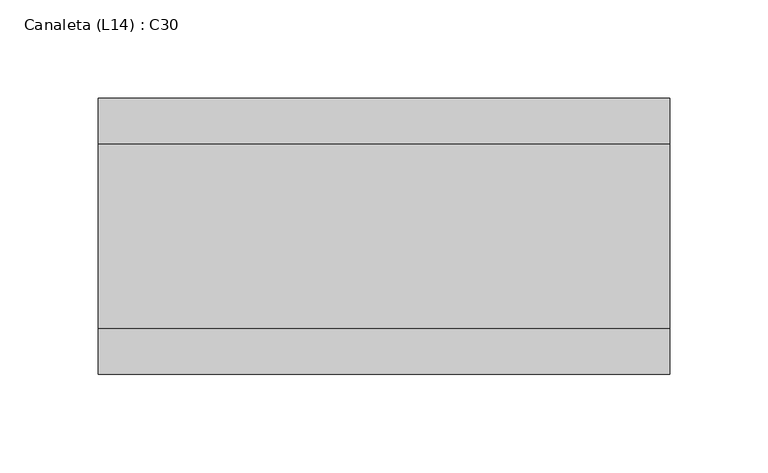
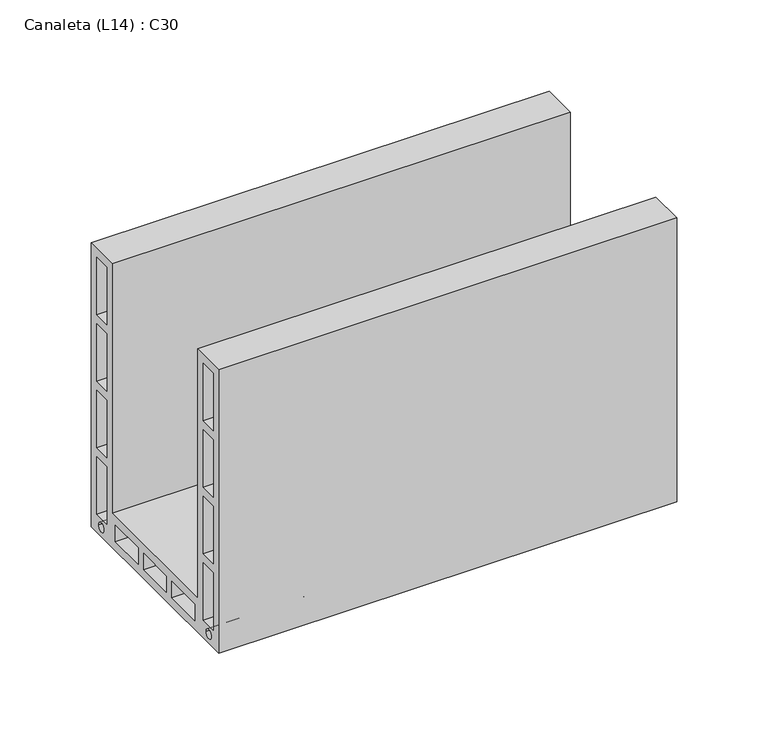
"""IFC4 building model written with IfcOpenShell, lengths in millimetres: proxy geometry, Canaleta (L14) : C30."""

from ifc_helpers import new_model, si_unit, point, frame, frame_2d, origin, place, context, project, spatial, polyline, circle_curve, trimmed, segment, composite_curve, outline, extrude, source, transform, mapped, element, save


def canaleta_l14_c30_f4fa639d(model_context):
    return source(origin(), model_context, "Body", "SweptSolid", [
        extrude(outline(polyline([(-140.0, 0.0), (-140.0, 190.0), (-117.0, 190.0), (-117.0, 23.0), (-23.0, 23.0), (-23.0, 190.0), (0.0, 190.0), (0.0, 0.0), (-140.0, 0.0)]), holes=[polyline([(-123.0, 184.0), (-134.0, 184.0), (-134.0, 145.5), (-123.0, 145.5), (-123.0, 184.0)]), polyline([(-123.0, 139.5), (-134.0, 139.5), (-134.0, 101.0), (-123.0, 101.0), (-123.0, 139.5)]), polyline([(-123.0, 95.0), (-134.0, 95.0), (-134.0, 56.5), (-123.0, 56.5), (-123.0, 95.0)]), polyline([(-123.0, 50.5), (-134.0, 50.5), (-134.0, 12.0), (-123.0, 12.0), (-123.0, 50.5)]), composite_curve([segment(trimmed(circle_curve(frame_2d((-128.9426557, 6.2112346)), 3.0), [point((-125.9426557, 6.2112346))], [point((-131.9426557, 6.2112346))], True, "CARTESIAN"), True, "CONTINUOUS"), segment(trimmed(circle_curve(frame_2d((-128.9426557, 6.2112346)), 3.0), [point((-131.9426557, 6.2112346))], [point((-125.9426557, 6.2112346))], True, "CARTESIAN"), True, "CONTINUOUS")], self_intersect=False), polyline([(-17.0, 184.0), (-17.0, 145.5), (-6.0, 145.5), (-6.0, 184.0), (-17.0, 184.0)]), polyline([(-17.0, 139.5), (-17.0, 101.0), (-6.0, 101.0), (-6.0, 139.5), (-17.0, 139.5)]), polyline([(-17.0, 95.0), (-17.0, 56.5), (-6.0, 56.5), (-6.0, 95.0), (-17.0, 95.0)]), polyline([(-17.0, 50.5), (-17.0, 12.0), (-6.0, 12.0), (-6.0, 50.5), (-17.0, 50.5)]), composite_curve([segment(trimmed(circle_curve(frame_2d((-11.0573443, 6.2112346)), 3.0), [point((-8.0573443, 6.2112346))], [point((-14.0573443, 6.2112346))], True, "CARTESIAN"), True, "CONTINUOUS"), segment(trimmed(circle_curve(frame_2d((-11.0573443, 6.2112346)), 3.0), [point((-14.0573443, 6.2112346))], [point((-8.0573443, 6.2112346))], True, "CARTESIAN"), True, "CONTINUOUS")], self_intersect=False), polyline([(-88.5, 17.0), (-113.5, 17.0), (-113.5, 6.0), (-88.5, 6.0), (-88.5, 17.0)]), polyline([(-57.5, 17.0), (-82.5, 17.0), (-82.5, 6.0), (-57.5, 6.0), (-57.5, 17.0)]), polyline([(-26.5, 17.0), (-51.5, 17.0), (-51.5, 6.0), (-26.5, 6.0), (-26.5, 17.0)])]), frame((0.0, 0.0, 0.0), z_axis=(1.0, 0.0, 0.0), x_axis=(0.0, 1.0, 0.0)), (0.0, 0.0, 1.0), 290.0),
    ])


if __name__ == "__main__":
    model = new_model("IFC4")
    model_context = context("Model", 3, world=origin())
    ifc_project = project(units=[si_unit("LENGTHUNIT", "METRE", prefix="MILLI")], contexts=[model_context])
    site = spatial("IfcSite", under=ifc_project)
    building = spatial("IfcBuilding", under=site)
    placement = place(None, origin())
    canaleta_l14_c30_shape = canaleta_l14_c30_f4fa639d(model_context)
    element("IfcBuildingElementProxy", 1, Name="Canaleta (L14) : C30", ObjectType="Canaleta (L14) : C30", at=placement, inside=building, context=model_context, shape_type="MappedRepresentation", body=[
        mapped(canaleta_l14_c30_shape, transform((0.0, 0.0, 0.0), x_axis=(1.0, 0.0, 0.0), y_axis=(0.0, 1.0, 0.0), z_axis=(0.0, 0.0, 1.0))),
    ])
    save(model, "model.ifc")

# Revit data of these elements
# Type "Canaleta (L14) : C30"
#   Comprimento = 0.290 m
#   Material [instance default] = Blocos Cerâmicos
#   Default Elevation = 0
# Element 1 (IfcBuildingElementProxy, "Canaleta (L14) : C30")
#   Materials on its faces: "Blocos Cerâmicos"
# Materials
#   "Blocos Cerâmicos": class "Genérico", colour RGB 177 84 47, transparency 0, Cost = 0
